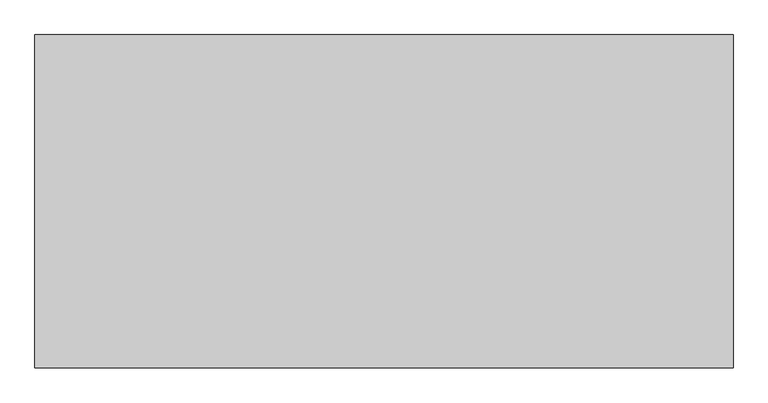
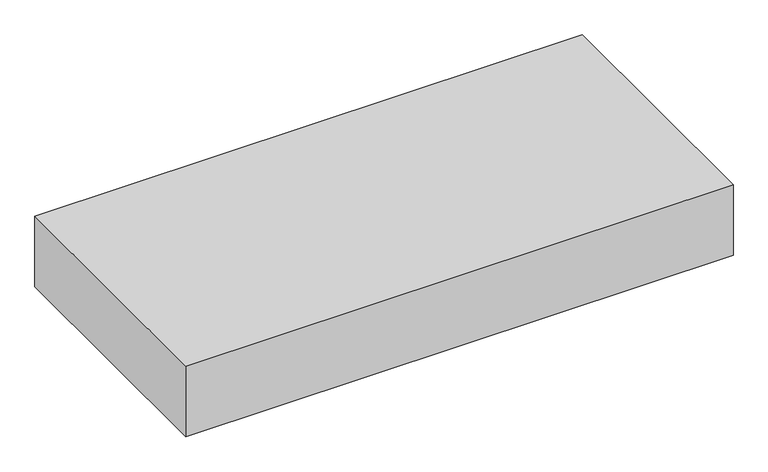
"""IFC4 building model written with IfcOpenShell, lengths in millimetres: proxy geometry, Space Planning Box_hec : Space Planning Box_hec."""

import ifcopenshell
import ifcopenshell.guid

model = None  # the IFC model being written
_history = None  # IfcOwnerHistory: only IFC2X3 demands one
_inside = {}  # id of a spatial element -> (the spatial element, [elements in it])
_under = {}  # id of a project, library or spatial element -> (it, [spatial elements below it])
_declared = {}  # id of a project -> (the project, [libraries it declares])
_typed = {}  # id of a type object -> (the type object, [elements of that type])
_made_of = {}  # id of a material, layer set ... -> (it, [elements and type objects made of it])


def new_model(schema):
    """Start an empty IFC model of exactly this schema.

    Asked for "IFC4X3", IfcOpenShell would pick the latest addendum, in which some entities
    have other attributes; the version numbers below select the first issue.
    IFC2X3 requires an IfcOwnerHistory on every rooted entity: one is made here for all.
    """
    global model, _history
    if schema == "IFC4X3":
        model = ifcopenshell.file(schema_version=(4, 3, 0, 0))
    else:
        model = ifcopenshell.file(schema=schema)
    _inside.clear()
    _under.clear()
    _declared.clear()
    _typed.clear()
    _made_of.clear()
    _history = None
    if model.schema == "IFC2X3":
        org = make("IfcOrganization", Name="unknown")
        user = make(
            "IfcPersonAndOrganization",
            ThePerson=make("IfcPerson", FamilyName="unknown"),
            TheOrganization=org,
        )
        app = make(
            "IfcApplication",
            ApplicationDeveloper=org,
            Version="unknown",
            ApplicationFullName="unknown",
            ApplicationIdentifier="unknown",
        )
        _history = make(
            "IfcOwnerHistory",
            OwningUser=user,
            OwningApplication=app,
            ChangeAction="ADDED",
            CreationDate=0,
        )
    return model


def make(cls, **values):
    """One entity of the class cls with the attributes given. An attribute that is None is left unset."""
    return model.create_entity(
        cls, **{name: value for name, value in values.items() if value is not None}
    )


def rooted(cls, **values):
    """An entity with a GlobalId (a new one), such as an element, a storey or a relation."""
    return make(cls, GlobalId=ifcopenshell.guid.new(), OwnerHistory=_history, **values)


def si_unit(unit_type, name, prefix=None):
    """IfcSIUnit, for example si_unit("LENGTHUNIT", "METRE", prefix="MILLI")."""
    return make("IfcSIUnit", UnitType=unit_type, Prefix=prefix, Name=name)


def assignment(units):
    """IfcUnitAssignment: the units of a project."""
    return None if units is None else make("IfcUnitAssignment", Units=units)


def point(xyz):
    """IfcCartesianPoint."""
    return None if xyz is None else make("IfcCartesianPoint", Coordinates=xyz)


def direction(xyz):
    """IfcDirection."""
    return None if xyz is None else make("IfcDirection", DirectionRatios=xyz)


def frame(location, z_axis=None, x_axis=None):
    """IfcAxis2Placement3D, a coordinate frame: its origin and axes. An axis left out is left unset."""
    return make(
        "IfcAxis2Placement3D",
        Location=point(location),
        Axis=direction(z_axis),
        RefDirection=direction(x_axis),
    )


def origin():
    """The frame at (0, 0, 0) with its axes left unset."""
    return frame((0.0, 0.0, 0.0))


def origin_with_axes():
    """The frame at (0, 0, 0) with the z axis (0, 0, 1) and the x axis (1, 0, 0) written out."""
    return frame((0.0, 0.0, 0.0), z_axis=(0.0, 0.0, 1.0), x_axis=(1.0, 0.0, 0.0))


def place(relative_to, where):
    """IfcLocalPlacement: puts the frame where relative to a parent placement (None: the world)."""
    return make(
        "IfcLocalPlacement", PlacementRelTo=relative_to, RelativePlacement=where
    )


def context(
    kind, dimensions, precision=None, world=None, true_north=None, identifier=None
):
    """IfcGeometricRepresentationContext, for example the 3D "Model" context."""
    return make(
        "IfcGeometricRepresentationContext",
        ContextIdentifier=identifier,
        ContextType=kind,
        CoordinateSpaceDimension=dimensions,
        Precision=precision,
        WorldCoordinateSystem=world,
        TrueNorth=true_north,
    )


def project(units=None, contexts=None):
    """IfcProject with its units and contexts."""
    return rooted(
        "IfcProject",
        Name="project",
        RepresentationContexts=contexts,
        UnitsInContext=assignment(units),
    )


def spatial(cls, under=None, at=None, **own):
    """A site, building, storey or space (cls), placed at a placement, below another one or the project."""
    s = rooted(cls, ObjectPlacement=at, **own)
    if under is not None:
        _under.setdefault(under.id(), (under, []))[1].append(s)
    return s


def polyline(points):
    """IfcPolyline through the points."""
    return make("IfcPolyline", Points=[point(p) for p in points])


def outline(outer, holes=None, kind="AREA"):
    """IfcArbitraryClosedProfileDef: a profile drawn as a closed curve; with holes, ...WithVoids."""
    if holes is None:
        return make("IfcArbitraryClosedProfileDef", ProfileType=kind, OuterCurve=outer)
    return make(
        "IfcArbitraryProfileDefWithVoids",
        ProfileType=kind,
        OuterCurve=outer,
        InnerCurves=holes,
    )


def extrude(swept, where, along, depth):
    """IfcExtrudedAreaSolid: the profile swept, set in the frame where, extruded along a direction by depth."""
    return make(
        "IfcExtrudedAreaSolid",
        SweptArea=swept,
        Position=where,
        ExtrudedDirection=direction(along),
        Depth=depth,
    )


def shape(context_of_items, identifier, shape_type, items):
    """IfcShapeRepresentation: the items that make up one representation, for example the "Body"."""
    return make(
        "IfcShapeRepresentation",
        ContextOfItems=context_of_items,
        RepresentationIdentifier=identifier,
        RepresentationType=shape_type,
        Items=items,
    )


def source(mapping_origin, context_of_items, identifier, shape_type, items):
    """IfcRepresentationMap: a shape defined once, which mapped items show again and again."""
    return make(
        "IfcRepresentationMap",
        MappingOrigin=mapping_origin,
        MappedRepresentation=shape(context_of_items, identifier, shape_type, items),
    )


def transform(
    local_origin,
    x_axis=None,
    y_axis=None,
    z_axis=None,
    scale=None,
    scale2=None,
    scale3=None,
    uniform=True,
):
    """IfcCartesianTransformationOperator3D, or its non-uniform kind. x_axis, y_axis, z_axis: its Axis1, 2, 3."""
    if uniform:
        return make(
            "IfcCartesianTransformationOperator3D",
            Axis1=direction(x_axis),
            Axis2=direction(y_axis),
            LocalOrigin=point(local_origin),
            Scale=scale,
            Axis3=direction(z_axis),
        )
    return make(
        "IfcCartesianTransformationOperator3DnonUniform",
        Axis1=direction(x_axis),
        Axis2=direction(y_axis),
        LocalOrigin=point(local_origin),
        Scale=scale,
        Axis3=direction(z_axis),
        Scale2=scale2,
        Scale3=scale3,
    )


def mapped(mapping_source, mapping_target):
    """IfcMappedItem: shows the shape of a source again, moved by a transform."""
    return make(
        "IfcMappedItem", MappingSource=mapping_source, MappingTarget=mapping_target
    )


def made_of(thing, what):
    """Note that an element or type object is made of a material, layer set ...; save() writes the relation."""
    if what is not None:
        _made_of.setdefault(what.id(), (what, []))[1].append(thing)
    return thing


def element(
    cls,
    number,
    at=None,
    inside=None,
    cuts=None,
    type_object=None,
    material=None,
    context=None,
    identifier="Body",
    shape_type=None,
    held_by="IfcProductDefinitionShape",
    body=None,
    shapes=None,
    **own,
):
    """One element of the class cls, such as IfcWall. Its Tag is "e" and its number.

    at: its placement. inside: the storey or other place that contains it. cuts: it is an
    opening in that element (IfcRelVoidsElement). A single representation is given by context,
    identifier, shape_type and body (its items); several are given by shapes. held_by: the class
    of the entity that holds the representations. save() writes the other relations.
    """
    e = rooted(cls, Tag="e%d" % number, ObjectPlacement=at, **own)
    if body is not None:
        shapes = [shape(context, identifier, shape_type, body)]
    if shapes is not None:
        e.Representation = make(held_by, Representations=shapes)
    if inside is not None:
        _inside.setdefault(inside.id(), (inside, []))[1].append(e)
    if cuts is not None:
        rooted(
            "IfcRelVoidsElement", RelatingBuildingElement=cuts, RelatedOpeningElement=e
        )
    if type_object is not None:
        _typed.setdefault(type_object.id(), (type_object, []))[1].append(e)
    return made_of(e, material)


def aggregate(whole, parts):
    """IfcRelAggregates: a whole, such as a stair, and the parts it consists of."""
    return rooted("IfcRelAggregates", RelatingObject=whole, RelatedObjects=parts)


def save(model, path):
    """Write the relations noted so far, then the file.

    IfcRelAggregates (storeys below a building ...), IfcRelContainedInSpatialStructure (elements
    in a storey), IfcRelDefinesByType, IfcRelAssociatesMaterial and IfcRelDeclares: one each for
    every whole, place, type object, material and project.
    """
    for whole, parts in _under.values():
        aggregate(whole, parts)
    for where, things in _inside.values():
        rooted(
            "IfcRelContainedInSpatialStructure",
            RelatedElements=things,
            RelatingStructure=where,
        )
    for kind, things in _typed.values():
        rooted("IfcRelDefinesByType", RelatedObjects=things, RelatingType=kind)
    for what, things in _made_of.values():
        rooted("IfcRelAssociatesMaterial", RelatedObjects=things, RelatingMaterial=what)
    for by, libraries in _declared.values():
        rooted("IfcRelDeclares", RelatingContext=by, RelatedDefinitions=libraries)
    model.write(path)


def generic_models_7e8091d6(model_context):
    return source(origin(), model_context, "Body", "SweptSolid", [
        extrude(outline(polyline([(22000.0, 10500.0), (22000.0, -10500.0), (-22000.0, -10500.0), (-22000.0, 10500.0), (22000.0, 10500.0)])), origin_with_axes(), (0.0, 0.0, 1.0), 6000.0),
    ])


if __name__ == "__main__":
    model = new_model("IFC4")
    model_context = context("Model", 3, world=origin())
    ifc_project = project(units=[si_unit("LENGTHUNIT", "METRE", prefix="MILLI")], contexts=[model_context])
    site = spatial("IfcSite", under=ifc_project)
    building = spatial("IfcBuilding", under=site)
    placement = place(None, origin())
    generic_models_shape = generic_models_7e8091d6(model_context)
    element("IfcBuildingElementProxy", 1, Name="Space Planning Box_hec : Space Planning Box_hec", ObjectType="Space Planning Box_hec : Space Planning Box_hec", at=placement, inside=building, context=model_context, shape_type="MappedRepresentation", body=[
        mapped(generic_models_shape, transform((0.0, 0.0, 0.0), x_axis=(1.0, 0.0, 0.0), y_axis=(0.0, 1.0, 0.0), z_axis=(0.0, 0.0, 1.0))),
    ])
    save(model, "model.ifc")

# Revit data of these elements
# Type "Space Planning Box_hec : Space Planning Box_hec"
#   Type Comments = "..."
#   Room Name [instance default] = "?"
#   Interior Finish [instance default] = ""
#   Exterior Finish [instance default] = ""
#   Department [instance default] = ""
#   Assembly Code = "..."
#   Width [instance default] = 1524 mm
#   Program Area [instance default] = 0.00 m²
#   Length [instance default] = 1524 mm
#   Height [instance default] = 1524 mm
#   Area [instance default] = 2.32258 m²
#   Fill Color [instance default] = Cyan
#   Default Elevation = 0
# Element 1 (IfcBuildingElementProxy, "Space Planning Box_hec : Space Planning Box_hec")
#   Room Name = "Corridor"
#   Interior Finish = "IF2-1"
#   Exterior Finish = "EF1"
#   Department = "AR"
#   Width = 44000 mm
#   Length = 21000 mm
#   Height = 6000 mm
#   Area = 924.00 m²
#   Fill Color = Lavender
#   Materials on its faces: "Lavender"
# Materials
#   "Cyan": class "Generic", colour RGB 0 255 255, transparency 0.2, Cost = 0
#   "Lavender": class "Generic", colour RGB 186 85 211, transparency 0.2, Cost = 0
